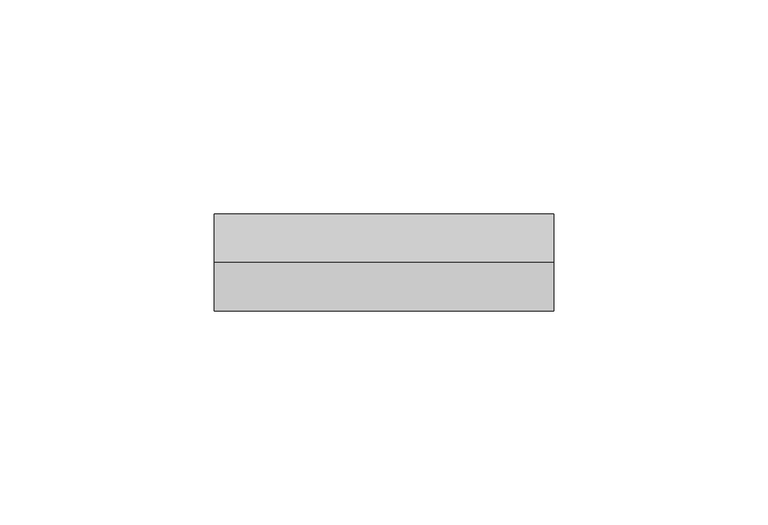
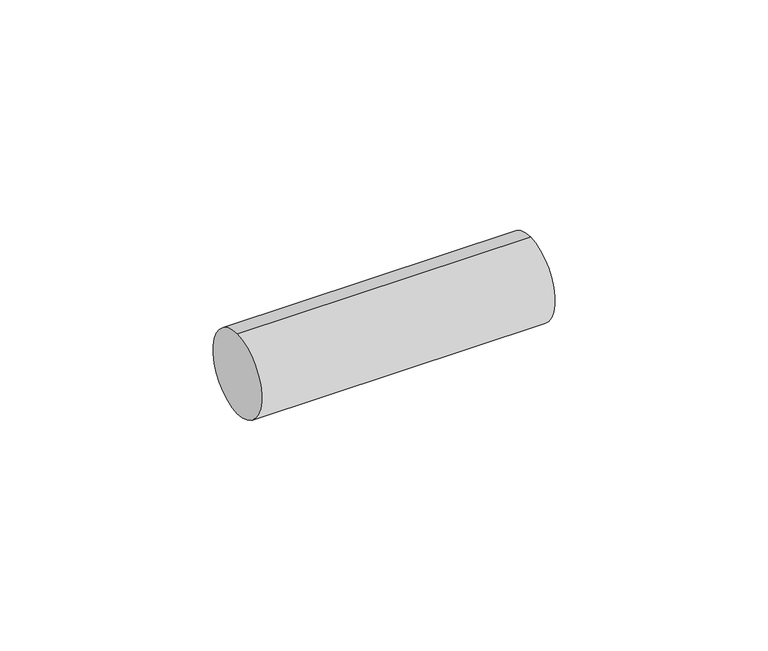
"""IFC4 building model written with IfcOpenShell, lengths in millimetres: proxy geometry, Bolt30:Bolt003:304751 : Bolt30:Bolt003:304751."""

from ifc_helpers import new_model, si_unit, point, frame, frame_2d, origin, place, context, project, spatial, circle_curve, trimmed, segment, composite_curve, outline, extrude, source, transform, mapped, element, save


def generic_models_79e5bdef(model_context):
    return source(origin(), model_context, "Body", "SweptSolid", [
        extrude(outline(composite_curve([segment(trimmed(circle_curve(frame_2d((2264.1630212, 39960.0063132)), 11.4045168), [point((2264.1630212, 39971.41083))], [point((2264.1630212, 39948.6017964))], False, "CARTESIAN"), True, "CONTINUOUS"), segment(trimmed(circle_curve(frame_2d((2264.1630212, 39960.0063132)), 11.4045168), [point((2264.1630212, 39948.6017964))], [point((2264.1630212, 39971.41083))], False, "CARTESIAN"), True, "CONTINUOUS")], self_intersect=False)), frame((15042.0981889, 0.0, 0.0), z_axis=(1.0, 0.0, 0.0), x_axis=(0.0, 1.0, 0.0)), (0.0, 0.0, 1.0), 79.375),
    ])


if __name__ == "__main__":
    model = new_model("IFC4")
    model_context = context("Model", 3, world=origin())
    ifc_project = project(units=[si_unit("LENGTHUNIT", "METRE", prefix="MILLI")], contexts=[model_context])
    site = spatial("IfcSite", under=ifc_project)
    building = spatial("IfcBuilding", under=site)
    placement = place(None, origin())
    generic_models_shape = generic_models_79e5bdef(model_context)
    element("IfcBuildingElementProxy", 1, Name="Bolt30:Bolt003:304751 : Bolt30:Bolt003:304751", ObjectType="Bolt30:Bolt003:304751 : Bolt30:Bolt003:304751", at=placement, inside=building, context=model_context, shape_type="MappedRepresentation", body=[
        mapped(generic_models_shape, transform((0.0, 0.0, 0.0), x_axis=(1.0, 0.0, 0.0), y_axis=(0.0, 1.0, 0.0), z_axis=(0.0, 0.0, 1.0))),
    ])
    save(model, "model.ifc")

# Revit data of these elements
# Type "Bolt30:Bolt003:304751 : Bolt30:Bolt003:304751"
#   NameOverride = "Bolt30:Bolt003:304751"
#   ObjectTypeOverride = "Bolt30:Bolt003"
#   Reference = "Bolt003"
#   Category = "Generic Models"
#   Tag = "304751"
# Element 1 (IfcBuildingElementProxy, "Bolt30:Bolt003:304751 : Bolt30:Bolt003:304751")
#   Materials on its faces: "TUBE STEEL STRINGER WELDED TO ANCHORED STEEL PLATE - SEE STRUCT DWGS"
# Materials
#   "TUBE STEEL STRINGER WELDED TO ANCHORED STEEL PLATE - SEE STRUCT DWGS": class "Unassigned", colour RGB 128 128 128, transparency 0, Cost = 0
